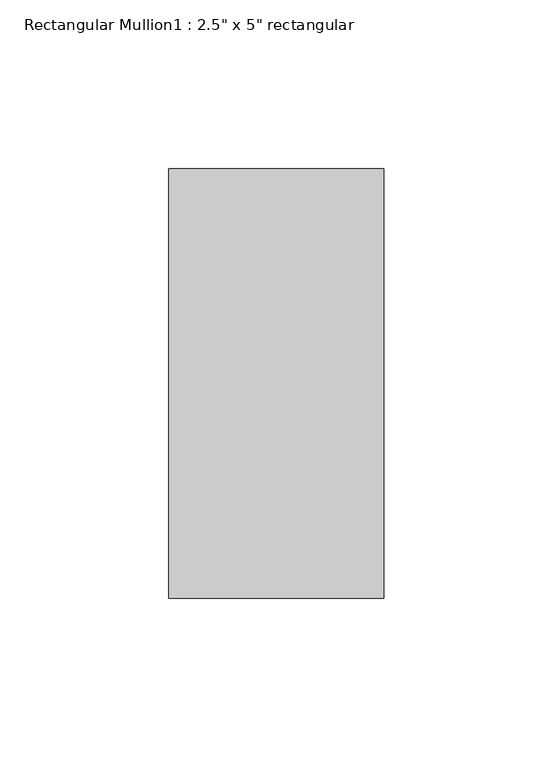
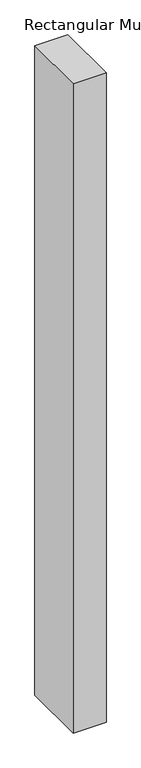
"""IFC4 building model written with IfcOpenShell, lengths in millimetres: member geometry."""

from ifc_helpers import new_model, si_unit, frame, origin, place, context, project, spatial, polyline, outline, extrude, source, transform, mapped, element, save


def member_f8a9089e(model_context):
    return source(origin(), model_context, "Body", "SweptSolid", [
        extrude(outline(polyline([(0.0, 63.5), (0.0, -63.5), (-63.5, -63.5), (-63.5, 63.5), (0.0, 63.5)])), frame((0.0, 0.0, -1320.067308), z_axis=(0.0, 0.0, 1.0), x_axis=(1.0, 0.0, 0.0)), (0.0, 0.0, 1.0), 1320.067308),
    ])


if __name__ == "__main__":
    model = new_model("IFC4")
    model_context = context("Model", 3, world=origin())
    ifc_project = project(units=[si_unit("LENGTHUNIT", "METRE", prefix="MILLI")], contexts=[model_context])
    site = spatial("IfcSite", under=ifc_project)
    building = spatial("IfcBuilding", under=site)
    placement = place(None, origin())
    member_shape = member_f8a9089e(model_context)
    element("IfcMember", 1, ObjectType="Rectangular Mullion1 : 2.5\" x 5\" rectangular", at=placement, inside=building, context=model_context, shape_type="MappedRepresentation", body=[
        mapped(member_shape, transform((0.0, 0.0, 0.0), x_axis=(1.0, 0.0, 0.0), y_axis=(0.0, 1.0, 0.0), z_axis=(0.0, 0.0, 1.0))),
    ])
    save(model, "model.ifc")

# Revit data of these elements
# Type "Rectangular Mullion1 : 2.5\" x 5\" rectangular"
#   built-in parameter 1007304 = 0.416667 (stored number, unit not read)
#   built-in parameter 1007301 = 0.104167 (stored number, unit not read)
#   built-in parameter 1007300 = 0.104167 (stored number, unit not read)
# Element 1 (IfcMember, "Rectangular Mullion1 : 2.5\" x 5\" rectangular")
#   Materials on its faces: "support-frame"
# Materials
#   "support-frame": class "Unassigned", colour RGB 233 233 233, transparency 0, Cost = 0
